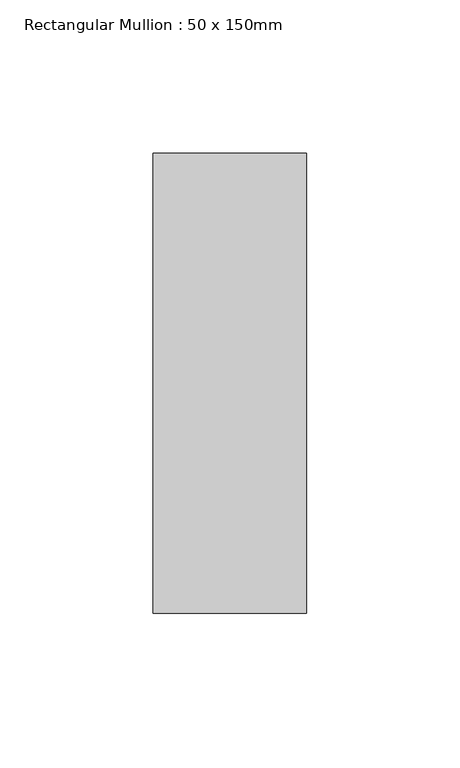
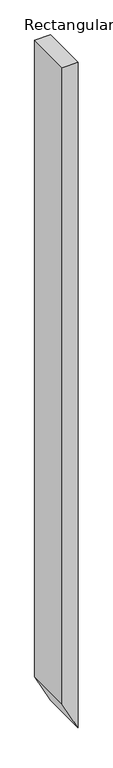
"""IFC4 building model written with IfcOpenShell, lengths in millimetres: member geometry, Rectangular Mullion : 50 x 150mm."""

import ifcopenshell
import ifcopenshell.guid

model = None  # the IFC model being written
_history = None  # IfcOwnerHistory: only IFC2X3 demands one
_inside = {}  # id of a spatial element -> (the spatial element, [elements in it])
_under = {}  # id of a project, library or spatial element -> (it, [spatial elements below it])
_declared = {}  # id of a project -> (the project, [libraries it declares])
_typed = {}  # id of a type object -> (the type object, [elements of that type])
_made_of = {}  # id of a material, layer set ... -> (it, [elements and type objects made of it])


def new_model(schema):
    """Start an empty IFC model of exactly this schema.

    Asked for "IFC4X3", IfcOpenShell would pick the latest addendum, in which some entities
    have other attributes; the version numbers below select the first issue.
    IFC2X3 requires an IfcOwnerHistory on every rooted entity: one is made here for all.
    """
    global model, _history
    if schema == "IFC4X3":
        model = ifcopenshell.file(schema_version=(4, 3, 0, 0))
    else:
        model = ifcopenshell.file(schema=schema)
    _inside.clear()
    _under.clear()
    _declared.clear()
    _typed.clear()
    _made_of.clear()
    _history = None
    if model.schema == "IFC2X3":
        org = make("IfcOrganization", Name="unknown")
        user = make(
            "IfcPersonAndOrganization",
            ThePerson=make("IfcPerson", FamilyName="unknown"),
            TheOrganization=org,
        )
        app = make(
            "IfcApplication",
            ApplicationDeveloper=org,
            Version="unknown",
            ApplicationFullName="unknown",
            ApplicationIdentifier="unknown",
        )
        _history = make(
            "IfcOwnerHistory",
            OwningUser=user,
            OwningApplication=app,
            ChangeAction="ADDED",
            CreationDate=0,
        )
    return model


def make(cls, **values):
    """One entity of the class cls with the attributes given. An attribute that is None is left unset."""
    return model.create_entity(
        cls, **{name: value for name, value in values.items() if value is not None}
    )


def rooted(cls, **values):
    """An entity with a GlobalId (a new one), such as an element, a storey or a relation."""
    return make(cls, GlobalId=ifcopenshell.guid.new(), OwnerHistory=_history, **values)


def si_unit(unit_type, name, prefix=None):
    """IfcSIUnit, for example si_unit("LENGTHUNIT", "METRE", prefix="MILLI")."""
    return make("IfcSIUnit", UnitType=unit_type, Prefix=prefix, Name=name)


def assignment(units):
    """IfcUnitAssignment: the units of a project."""
    return None if units is None else make("IfcUnitAssignment", Units=units)


def point(xyz):
    """IfcCartesianPoint."""
    return None if xyz is None else make("IfcCartesianPoint", Coordinates=xyz)


def direction(xyz):
    """IfcDirection."""
    return None if xyz is None else make("IfcDirection", DirectionRatios=xyz)


def frame(location, z_axis=None, x_axis=None):
    """IfcAxis2Placement3D, a coordinate frame: its origin and axes. An axis left out is left unset."""
    return make(
        "IfcAxis2Placement3D",
        Location=point(location),
        Axis=direction(z_axis),
        RefDirection=direction(x_axis),
    )


def origin():
    """The frame at (0, 0, 0) with its axes left unset."""
    return frame((0.0, 0.0, 0.0))


def place(relative_to, where):
    """IfcLocalPlacement: puts the frame where relative to a parent placement (None: the world)."""
    return make(
        "IfcLocalPlacement", PlacementRelTo=relative_to, RelativePlacement=where
    )


def context(
    kind, dimensions, precision=None, world=None, true_north=None, identifier=None
):
    """IfcGeometricRepresentationContext, for example the 3D "Model" context."""
    return make(
        "IfcGeometricRepresentationContext",
        ContextIdentifier=identifier,
        ContextType=kind,
        CoordinateSpaceDimension=dimensions,
        Precision=precision,
        WorldCoordinateSystem=world,
        TrueNorth=true_north,
    )


def project(units=None, contexts=None):
    """IfcProject with its units and contexts."""
    return rooted(
        "IfcProject",
        Name="project",
        RepresentationContexts=contexts,
        UnitsInContext=assignment(units),
    )


def spatial(cls, under=None, at=None, **own):
    """A site, building, storey or space (cls), placed at a placement, below another one or the project."""
    s = rooted(cls, ObjectPlacement=at, **own)
    if under is not None:
        _under.setdefault(under.id(), (under, []))[1].append(s)
    return s


def polyline(points):
    """IfcPolyline through the points."""
    return make("IfcPolyline", Points=[point(p) for p in points])


def outline(outer, holes=None, kind="AREA"):
    """IfcArbitraryClosedProfileDef: a profile drawn as a closed curve; with holes, ...WithVoids."""
    if holes is None:
        return make("IfcArbitraryClosedProfileDef", ProfileType=kind, OuterCurve=outer)
    return make(
        "IfcArbitraryProfileDefWithVoids",
        ProfileType=kind,
        OuterCurve=outer,
        InnerCurves=holes,
    )


def extrude(swept, where, along, depth):
    """IfcExtrudedAreaSolid: the profile swept, set in the frame where, extruded along a direction by depth."""
    return make(
        "IfcExtrudedAreaSolid",
        SweptArea=swept,
        Position=where,
        ExtrudedDirection=direction(along),
        Depth=depth,
    )


def shape(context_of_items, identifier, shape_type, items):
    """IfcShapeRepresentation: the items that make up one representation, for example the "Body"."""
    return make(
        "IfcShapeRepresentation",
        ContextOfItems=context_of_items,
        RepresentationIdentifier=identifier,
        RepresentationType=shape_type,
        Items=items,
    )


def source(mapping_origin, context_of_items, identifier, shape_type, items):
    """IfcRepresentationMap: a shape defined once, which mapped items show again and again."""
    return make(
        "IfcRepresentationMap",
        MappingOrigin=mapping_origin,
        MappedRepresentation=shape(context_of_items, identifier, shape_type, items),
    )


def transform(
    local_origin,
    x_axis=None,
    y_axis=None,
    z_axis=None,
    scale=None,
    scale2=None,
    scale3=None,
    uniform=True,
):
    """IfcCartesianTransformationOperator3D, or its non-uniform kind. x_axis, y_axis, z_axis: its Axis1, 2, 3."""
    if uniform:
        return make(
            "IfcCartesianTransformationOperator3D",
            Axis1=direction(x_axis),
            Axis2=direction(y_axis),
            LocalOrigin=point(local_origin),
            Scale=scale,
            Axis3=direction(z_axis),
        )
    return make(
        "IfcCartesianTransformationOperator3DnonUniform",
        Axis1=direction(x_axis),
        Axis2=direction(y_axis),
        LocalOrigin=point(local_origin),
        Scale=scale,
        Axis3=direction(z_axis),
        Scale2=scale2,
        Scale3=scale3,
    )


def mapped(mapping_source, mapping_target):
    """IfcMappedItem: shows the shape of a source again, moved by a transform."""
    return make(
        "IfcMappedItem", MappingSource=mapping_source, MappingTarget=mapping_target
    )


def made_of(thing, what):
    """Note that an element or type object is made of a material, layer set ...; save() writes the relation."""
    if what is not None:
        _made_of.setdefault(what.id(), (what, []))[1].append(thing)
    return thing


def element(
    cls,
    number,
    at=None,
    inside=None,
    cuts=None,
    type_object=None,
    material=None,
    context=None,
    identifier="Body",
    shape_type=None,
    held_by="IfcProductDefinitionShape",
    body=None,
    shapes=None,
    **own,
):
    """One element of the class cls, such as IfcWall. Its Tag is "e" and its number.

    at: its placement. inside: the storey or other place that contains it. cuts: it is an
    opening in that element (IfcRelVoidsElement). A single representation is given by context,
    identifier, shape_type and body (its items); several are given by shapes. held_by: the class
    of the entity that holds the representations. save() writes the other relations.
    """
    e = rooted(cls, Tag="e%d" % number, ObjectPlacement=at, **own)
    if body is not None:
        shapes = [shape(context, identifier, shape_type, body)]
    if shapes is not None:
        e.Representation = make(held_by, Representations=shapes)
    if inside is not None:
        _inside.setdefault(inside.id(), (inside, []))[1].append(e)
    if cuts is not None:
        rooted(
            "IfcRelVoidsElement", RelatingBuildingElement=cuts, RelatedOpeningElement=e
        )
    if type_object is not None:
        _typed.setdefault(type_object.id(), (type_object, []))[1].append(e)
    return made_of(e, material)


def aggregate(whole, parts):
    """IfcRelAggregates: a whole, such as a stair, and the parts it consists of."""
    return rooted("IfcRelAggregates", RelatingObject=whole, RelatedObjects=parts)


def save(model, path):
    """Write the relations noted so far, then the file.

    IfcRelAggregates (storeys below a building ...), IfcRelContainedInSpatialStructure (elements
    in a storey), IfcRelDefinesByType, IfcRelAssociatesMaterial and IfcRelDeclares: one each for
    every whole, place, type object, material and project.
    """
    for whole, parts in _under.values():
        aggregate(whole, parts)
    for where, things in _inside.values():
        rooted(
            "IfcRelContainedInSpatialStructure",
            RelatedElements=things,
            RelatingStructure=where,
        )
    for kind, things in _typed.values():
        rooted("IfcRelDefinesByType", RelatedObjects=things, RelatingType=kind)
    for what, things in _made_of.values():
        rooted("IfcRelAssociatesMaterial", RelatedObjects=things, RelatingMaterial=what)
    for by, libraries in _declared.values():
        rooted("IfcRelDeclares", RelatingContext=by, RelatedDefinitions=libraries)
    model.write(path)


def rectangular_mullion_50_x_150mm_2f01cdb9(model_context):
    return source(origin(), model_context, "Body", "SweptSolid", [
        extrude(outline(polyline([(0.0, 0.0), (0.0, -50.0), (-2114.4282315, -50.0), (-2210.4773379, 0.0), (0.0, 0.0)])), frame((0.0, -75.0, 0.0), z_axis=(0.0, 1.0, 0.0), x_axis=(0.0, 0.0, 1.0)), (0.0, 0.0, 1.0), 150.0),
    ])


if __name__ == "__main__":
    model = new_model("IFC4")
    model_context = context("Model", 3, world=origin())
    ifc_project = project(units=[si_unit("LENGTHUNIT", "METRE", prefix="MILLI")], contexts=[model_context])
    site = spatial("IfcSite", under=ifc_project)
    building = spatial("IfcBuilding", under=site)
    placement = place(None, origin())
    rectangular_mullion_50_x_150mm_shape = rectangular_mullion_50_x_150mm_2f01cdb9(model_context)
    element("IfcMember", 1, ObjectType="Rectangular Mullion : 50 x 150mm", at=placement, inside=building, context=model_context, shape_type="MappedRepresentation", body=[
        mapped(rectangular_mullion_50_x_150mm_shape, transform((0.0, 0.0, 0.0), x_axis=(1.0, 0.0, 0.0), y_axis=(0.0, 1.0, 0.0), z_axis=(0.0, 0.0, 1.0))),
    ])
    save(model, "model.ifc")

# Revit data of these elements
# Type "Rectangular Mullion : 50 x 150mm"
#   built-in parameter 1007304 = 0.492126 (stored number, unit not read)
#   built-in parameter 1007301 = 0.082021 (stored number, unit not read)
#   built-in parameter 1007300 = 0.082021 (stored number, unit not read)
# Element 1 (IfcMember, "Rectangular Mullion : 50 x 150mm")
#   Materials on its faces: "Aluminium"
# Materials
#   "Aluminium": class "Metal", colour RGB 247 247 247, transparency 0, Description = "Aluminium 6061", Cost = 0
